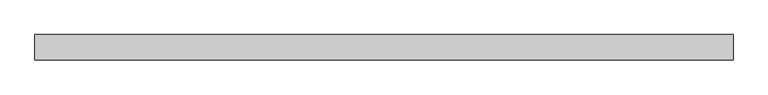
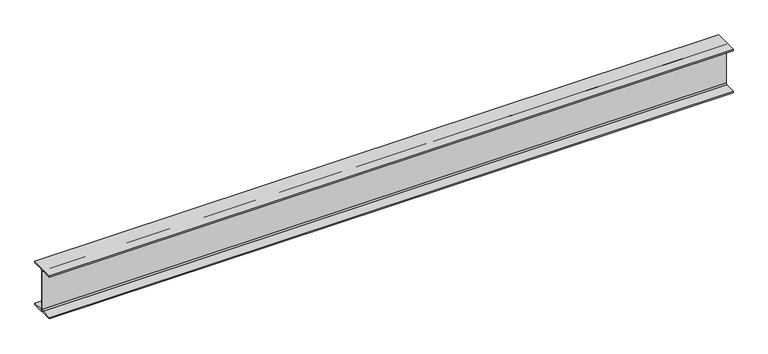
"""IFC4 building model written with IfcOpenShell, lengths in millimetres: beam geometry, Old_Steel Beam_H-KSD3502 : H_SB_ASB_H-250×125x6x9."""

import ifcopenshell
import ifcopenshell.guid

model = None  # the IFC model being written
_history = None  # IfcOwnerHistory: only IFC2X3 demands one
_inside = {}  # id of a spatial element -> (the spatial element, [elements in it])
_under = {}  # id of a project, library or spatial element -> (it, [spatial elements below it])
_declared = {}  # id of a project -> (the project, [libraries it declares])
_typed = {}  # id of a type object -> (the type object, [elements of that type])
_made_of = {}  # id of a material, layer set ... -> (it, [elements and type objects made of it])


def new_model(schema):
    """Start an empty IFC model of exactly this schema.

    Asked for "IFC4X3", IfcOpenShell would pick the latest addendum, in which some entities
    have other attributes; the version numbers below select the first issue.
    IFC2X3 requires an IfcOwnerHistory on every rooted entity: one is made here for all.
    """
    global model, _history
    if schema == "IFC4X3":
        model = ifcopenshell.file(schema_version=(4, 3, 0, 0))
    else:
        model = ifcopenshell.file(schema=schema)
    _inside.clear()
    _under.clear()
    _declared.clear()
    _typed.clear()
    _made_of.clear()
    _history = None
    if model.schema == "IFC2X3":
        org = make("IfcOrganization", Name="unknown")
        user = make(
            "IfcPersonAndOrganization",
            ThePerson=make("IfcPerson", FamilyName="unknown"),
            TheOrganization=org,
        )
        app = make(
            "IfcApplication",
            ApplicationDeveloper=org,
            Version="unknown",
            ApplicationFullName="unknown",
            ApplicationIdentifier="unknown",
        )
        _history = make(
            "IfcOwnerHistory",
            OwningUser=user,
            OwningApplication=app,
            ChangeAction="ADDED",
            CreationDate=0,
        )
    return model


def make(cls, **values):
    """One entity of the class cls with the attributes given. An attribute that is None is left unset."""
    return model.create_entity(
        cls, **{name: value for name, value in values.items() if value is not None}
    )


def rooted(cls, **values):
    """An entity with a GlobalId (a new one), such as an element, a storey or a relation."""
    return make(cls, GlobalId=ifcopenshell.guid.new(), OwnerHistory=_history, **values)


def si_unit(unit_type, name, prefix=None):
    """IfcSIUnit, for example si_unit("LENGTHUNIT", "METRE", prefix="MILLI")."""
    return make("IfcSIUnit", UnitType=unit_type, Prefix=prefix, Name=name)


def assignment(units):
    """IfcUnitAssignment: the units of a project."""
    return None if units is None else make("IfcUnitAssignment", Units=units)


def point(xyz):
    """IfcCartesianPoint."""
    return None if xyz is None else make("IfcCartesianPoint", Coordinates=xyz)


def direction(xyz):
    """IfcDirection."""
    return None if xyz is None else make("IfcDirection", DirectionRatios=xyz)


def frame(location, z_axis=None, x_axis=None):
    """IfcAxis2Placement3D, a coordinate frame: its origin and axes. An axis left out is left unset."""
    return make(
        "IfcAxis2Placement3D",
        Location=point(location),
        Axis=direction(z_axis),
        RefDirection=direction(x_axis),
    )


def frame_2d(location, x_axis=None):
    """IfcAxis2Placement2D, a coordinate frame in the plane: its origin and x axis."""
    return make(
        "IfcAxis2Placement2D", Location=point(location), RefDirection=direction(x_axis)
    )


def origin():
    """The frame at (0, 0, 0) with its axes left unset."""
    return frame((0.0, 0.0, 0.0))


def place(relative_to, where):
    """IfcLocalPlacement: puts the frame where relative to a parent placement (None: the world)."""
    return make(
        "IfcLocalPlacement", PlacementRelTo=relative_to, RelativePlacement=where
    )


def context(
    kind, dimensions, precision=None, world=None, true_north=None, identifier=None
):
    """IfcGeometricRepresentationContext, for example the 3D "Model" context."""
    return make(
        "IfcGeometricRepresentationContext",
        ContextIdentifier=identifier,
        ContextType=kind,
        CoordinateSpaceDimension=dimensions,
        Precision=precision,
        WorldCoordinateSystem=world,
        TrueNorth=true_north,
    )


def project(units=None, contexts=None):
    """IfcProject with its units and contexts."""
    return rooted(
        "IfcProject",
        Name="project",
        RepresentationContexts=contexts,
        UnitsInContext=assignment(units),
    )


def spatial(cls, under=None, at=None, **own):
    """A site, building, storey or space (cls), placed at a placement, below another one or the project."""
    s = rooted(cls, ObjectPlacement=at, **own)
    if under is not None:
        _under.setdefault(under.id(), (under, []))[1].append(s)
    return s


def polyline(points):
    """IfcPolyline through the points."""
    return make("IfcPolyline", Points=[point(p) for p in points])


def circle_curve(where, radius):
    """IfcCircle in the frame where."""
    return make("IfcCircle", Position=where, Radius=radius)


def trimmed(basis, trim1, trim2, sense, master):
    """IfcTrimmedCurve: the piece of a basis curve between two trims."""
    return make(
        "IfcTrimmedCurve",
        BasisCurve=basis,
        Trim1=trim1,
        Trim2=trim2,
        SenseAgreement=sense,
        MasterRepresentation=master,
    )


def segment(curve, same_sense, transition):
    """IfcCompositeCurveSegment."""
    return make(
        "IfcCompositeCurveSegment",
        Transition=transition,
        SameSense=same_sense,
        ParentCurve=curve,
    )


def composite_curve(segments, self_intersect=None):
    """IfcCompositeCurve: segments joined end to end."""
    return make("IfcCompositeCurve", Segments=segments, SelfIntersect=self_intersect)


def outline(outer, holes=None, kind="AREA"):
    """IfcArbitraryClosedProfileDef: a profile drawn as a closed curve; with holes, ...WithVoids."""
    if holes is None:
        return make("IfcArbitraryClosedProfileDef", ProfileType=kind, OuterCurve=outer)
    return make(
        "IfcArbitraryProfileDefWithVoids",
        ProfileType=kind,
        OuterCurve=outer,
        InnerCurves=holes,
    )


def extrude(swept, where, along, depth):
    """IfcExtrudedAreaSolid: the profile swept, set in the frame where, extruded along a direction by depth."""
    return make(
        "IfcExtrudedAreaSolid",
        SweptArea=swept,
        Position=where,
        ExtrudedDirection=direction(along),
        Depth=depth,
    )


def shape(context_of_items, identifier, shape_type, items):
    """IfcShapeRepresentation: the items that make up one representation, for example the "Body"."""
    return make(
        "IfcShapeRepresentation",
        ContextOfItems=context_of_items,
        RepresentationIdentifier=identifier,
        RepresentationType=shape_type,
        Items=items,
    )


def source(mapping_origin, context_of_items, identifier, shape_type, items):
    """IfcRepresentationMap: a shape defined once, which mapped items show again and again."""
    return make(
        "IfcRepresentationMap",
        MappingOrigin=mapping_origin,
        MappedRepresentation=shape(context_of_items, identifier, shape_type, items),
    )


def transform(
    local_origin,
    x_axis=None,
    y_axis=None,
    z_axis=None,
    scale=None,
    scale2=None,
    scale3=None,
    uniform=True,
):
    """IfcCartesianTransformationOperator3D, or its non-uniform kind. x_axis, y_axis, z_axis: its Axis1, 2, 3."""
    if uniform:
        return make(
            "IfcCartesianTransformationOperator3D",
            Axis1=direction(x_axis),
            Axis2=direction(y_axis),
            LocalOrigin=point(local_origin),
            Scale=scale,
            Axis3=direction(z_axis),
        )
    return make(
        "IfcCartesianTransformationOperator3DnonUniform",
        Axis1=direction(x_axis),
        Axis2=direction(y_axis),
        LocalOrigin=point(local_origin),
        Scale=scale,
        Axis3=direction(z_axis),
        Scale2=scale2,
        Scale3=scale3,
    )


def mapped(mapping_source, mapping_target):
    """IfcMappedItem: shows the shape of a source again, moved by a transform."""
    return make(
        "IfcMappedItem", MappingSource=mapping_source, MappingTarget=mapping_target
    )


def made_of(thing, what):
    """Note that an element or type object is made of a material, layer set ...; save() writes the relation."""
    if what is not None:
        _made_of.setdefault(what.id(), (what, []))[1].append(thing)
    return thing


def element(
    cls,
    number,
    at=None,
    inside=None,
    cuts=None,
    type_object=None,
    material=None,
    context=None,
    identifier="Body",
    shape_type=None,
    held_by="IfcProductDefinitionShape",
    body=None,
    shapes=None,
    **own,
):
    """One element of the class cls, such as IfcWall. Its Tag is "e" and its number.

    at: its placement. inside: the storey or other place that contains it. cuts: it is an
    opening in that element (IfcRelVoidsElement). A single representation is given by context,
    identifier, shape_type and body (its items); several are given by shapes. held_by: the class
    of the entity that holds the representations. save() writes the other relations.
    """
    e = rooted(cls, Tag="e%d" % number, ObjectPlacement=at, **own)
    if body is not None:
        shapes = [shape(context, identifier, shape_type, body)]
    if shapes is not None:
        e.Representation = make(held_by, Representations=shapes)
    if inside is not None:
        _inside.setdefault(inside.id(), (inside, []))[1].append(e)
    if cuts is not None:
        rooted(
            "IfcRelVoidsElement", RelatingBuildingElement=cuts, RelatedOpeningElement=e
        )
    if type_object is not None:
        _typed.setdefault(type_object.id(), (type_object, []))[1].append(e)
    return made_of(e, material)


def aggregate(whole, parts):
    """IfcRelAggregates: a whole, such as a stair, and the parts it consists of."""
    return rooted("IfcRelAggregates", RelatingObject=whole, RelatedObjects=parts)


def save(model, path):
    """Write the relations noted so far, then the file.

    IfcRelAggregates (storeys below a building ...), IfcRelContainedInSpatialStructure (elements
    in a storey), IfcRelDefinesByType, IfcRelAssociatesMaterial and IfcRelDeclares: one each for
    every whole, place, type object, material and project.
    """
    for whole, parts in _under.values():
        aggregate(whole, parts)
    for where, things in _inside.values():
        rooted(
            "IfcRelContainedInSpatialStructure",
            RelatedElements=things,
            RelatingStructure=where,
        )
    for kind, things in _typed.values():
        rooted("IfcRelDefinesByType", RelatedObjects=things, RelatingType=kind)
    for what, things in _made_of.values():
        rooted("IfcRelAssociatesMaterial", RelatedObjects=things, RelatingMaterial=what)
    for by, libraries in _declared.values():
        rooted("IfcRelDeclares", RelatingContext=by, RelatedDefinitions=libraries)
    model.write(path)


def beam_873fa0fc(model_context):
    return source(origin(), model_context, "Body", "SweptSolid", [
        extrude(outline(composite_curve([segment(polyline([(82.5, -141.5), (82.5, -151.7), (-82.5, -151.7), (-82.5, -141.5), (-11.9, -141.5)]), True, "CONTINUOUS"), segment(trimmed(circle_curve(frame_2d((-11.9, -132.6)), 8.9), [point((-11.9, -141.5))], [point((-3.0, -132.6))], True, "CARTESIAN"), True, "CONTINUOUS"), segment(polyline([(-3.0, -132.6), (-3.0, 132.6)]), True, "CONTINUOUS"), segment(trimmed(circle_curve(frame_2d((-11.9, 132.6)), 8.9), [point((-3.0, 132.6))], [point((-11.9, 141.5))], True, "CARTESIAN"), True, "CONTINUOUS"), segment(polyline([(-11.9, 141.5), (-82.5, 141.5), (-82.5, 151.7), (82.5, 151.7), (82.5, 141.5), (11.9, 141.5)]), True, "CONTINUOUS"), segment(trimmed(circle_curve(frame_2d((11.9, 132.6)), 8.9), [point((11.9, 141.5))], [point((3.0, 132.6))], True, "CARTESIAN"), True, "CONTINUOUS"), segment(polyline([(3.0, 132.6), (3.0, -132.6)]), True, "CONTINUOUS"), segment(trimmed(circle_curve(frame_2d((11.9, -132.6)), 8.9), [point((3.0, -132.6))], [point((11.9, -141.5))], True, "CARTESIAN"), True, "CONTINUOUS"), segment(polyline([(11.9, -141.5), (82.5, -141.5)]), True, "CONTINUOUS")], self_intersect=False)), frame((-2164.4729123, 0.0, 0.0), z_axis=(1.0, 0.0, 0.0), x_axis=(0.0, 1.0, 0.0)), (0.0, 0.0, 1.0), 4526.7729123),
    ])


if __name__ == "__main__":
    model = new_model("IFC4")
    model_context = context("Model", 3, world=origin())
    ifc_project = project(units=[si_unit("LENGTHUNIT", "METRE", prefix="MILLI")], contexts=[model_context])
    site = spatial("IfcSite", under=ifc_project)
    building = spatial("IfcBuilding", under=site)
    placement = place(None, origin())
    beam_shape = beam_873fa0fc(model_context)
    element("IfcBeam", 1, ObjectType="Old_Steel Beam_H-KSD3502 : H_SB_ASB_H-250×125x6x9", at=placement, inside=building, context=model_context, shape_type="MappedRepresentation", body=[
        mapped(beam_shape, transform((0.0, 0.0, 0.0), x_axis=(1.0, 0.0, 0.0), y_axis=(0.0, 1.0, 0.0), z_axis=(0.0, 0.0, 1.0))),
    ])
    save(model, "model.ifc")

# Revit data of these elements
# Type "Old_Steel Beam_H-KSD3502 : H_SB_ASB_H-250×125x6x9"
#   Width = 12.5 cm
#   Web Thickness = 0.6 cm
#   Web Fillet = 1.2 cm
#   Warping Constant = 42539.8 cm⁶
#   Torsional Moment of Inertia = 7.8102 cm⁴
#   Torsional Modulus = 1.0 cm³
#   Section Area = 37.66 cm²
#   Plastic Modulus weak axis = 73.1 cm³
#   Plastic Modulus strong axis = 366.0 cm³
#   Perimeter = 0.97 m²/m
#   Nominal Weight = 29.60 kgf/m
#   Moment of Inertia weak axis = 294.00 cm⁴
#   Moment of Inertia strong axis = 4050.00 cm⁴
#   Height = 25.0 cm
#   Flange Thickness = 0.9 cm
#   Elastic Modulus weak axis = 47.0 cm³
#   Elastic Modulus strong axis = 324.0 cm³
#   Centroid Vertical = 12.5 cm
#   Centroid Horizontal = 6.25 cm
#   Length [instance default] = 1.5240 m
#   Structural Material [instance default] = Steel, 45-345
#   Assembly Code = ""
# Element 1 (IfcBeam, "Old_Steel Beam_H-KSD3502 : H_SB_ASB_H-250×125x6x9")
#   Structural Material = none
# Materials
#   "Steel, 45-345": class "Metal", colour RGB 189 187 185, transparency 0, Description = "Steel 345 MPa", Cost = 0
